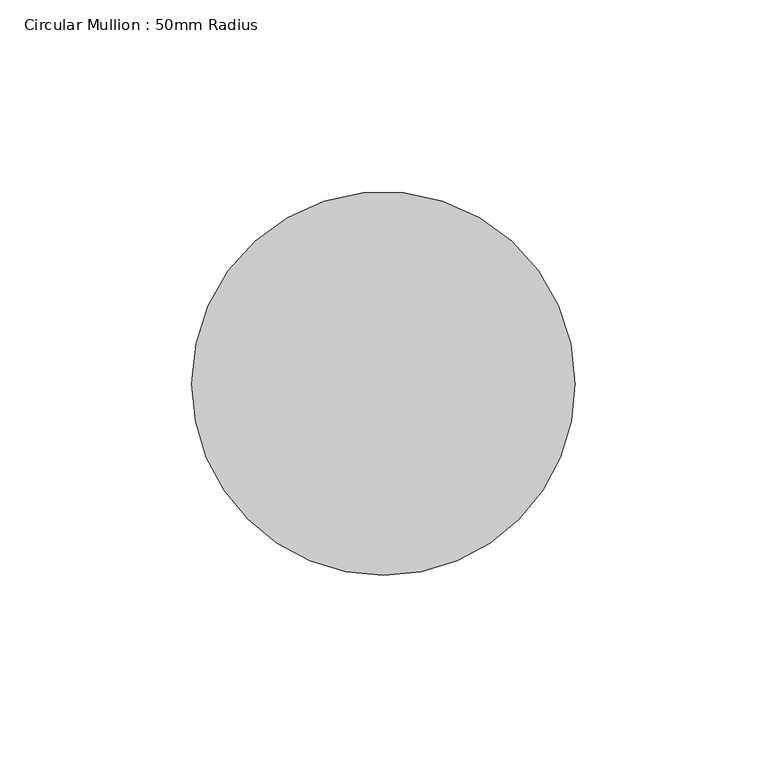
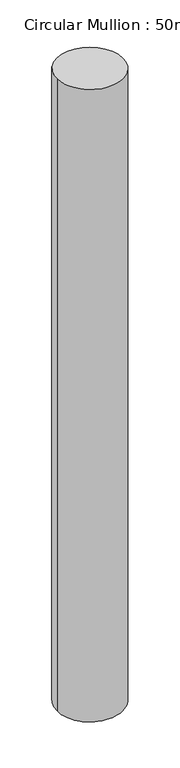
"""IFC4 building model written with IfcOpenShell, lengths in millimetres: member geometry, Circular Mullion : 50mm Radius."""

from ifc_helpers import new_model, si_unit, frame, origin, place, context, project, spatial, ellipse_curve, source, transform, mapped, element, save
from ifc_brep_helpers import plane_surface, cylinder_surface, advanced_brep


def circular_mullion_50mm_radius_8a95fe05(model_context):
    return source(origin(), model_context, "Body", "AdvancedBrep", [
        advanced_brep(
        [(-100.0, 0.0, 1.6217171), (0.0, 0.0, 0.0), (0.0, 0.0, -1012.0497266), (-100.0, 0.0, -1013.6442396)],
        [
            (0, 1, ellipse_curve(frame((-50.0, 0.0, 0.8108586), z_axis=(-0.01621331859733197, -0.014566336703536234, -0.9997624468518012), x_axis=(-0.7437023213754502, -0.6681555262929935, 0.021795638666932717)), 50.0118805, 50.0)),
            (1, 2),
            (2, 3, ellipse_curve(frame((-50.0, 0.0, -1012.8469831), z_axis=(-0.01594146823200777, -0.01432210145147921, 0.9997703471300905), x_axis=(0.7437081982268304, 0.6681608061618276, 0.021430188972056945)), 50.0114853, 50.0)),
            (3, 0),
            (1, 0, ellipse_curve(frame((-50.0, 0.0, 0.8108586), z_axis=(-0.01621331859733197, -0.014566336703536234, -0.9997624468518012), x_axis=(-0.7437023213754502, -0.6681555262929935, 0.021795638666932717)), 50.0118805, 50.0)),
            (3, 2, ellipse_curve(frame((-50.0, 0.0, -1012.8469831), z_axis=(-0.01594146823200777, -0.01432210145147921, 0.9997703471300905), x_axis=(0.7437081982268304, 0.6681608061618276, 0.021430188972056945)), 50.0114853, 50.0)),
        ],
        [
            cylinder_surface(frame((-50.0, 0.0, 0.0), z_axis=(0.0, 0.0, 1.0), x_axis=(1.0, 0.0, 0.0)), 50.0),
            plane_surface(frame((-203.7021945, 226.734329, 0.0), z_axis=(0.016213318597331973, 0.014566336703536237, 0.9997624468518014), x_axis=(0.7437023213754501, 0.6681555262929938, -0.02179563866693008))),
            plane_surface(frame((-203.7021945, 226.734329, -1012.0497266), z_axis=(0.01594146823200777, 0.01432210145147921, -0.9997703471300905), x_axis=(0.7437081982268302, 0.6681608061618275, 0.02143018897206872))),
        ],
        [
            (0, [[1, 2, 3, 4]]),
            (0, [[5, -4, 6, -2]]),
            (1, [[-1, -5]]),
            (2, [[-6, -3]]),
        ],
    ),
    ])


if __name__ == "__main__":
    model = new_model("IFC4")
    model_context = context("Model", 3, world=origin())
    ifc_project = project(units=[si_unit("LENGTHUNIT", "METRE", prefix="MILLI")], contexts=[model_context])
    site = spatial("IfcSite", under=ifc_project)
    building = spatial("IfcBuilding", under=site)
    placement = place(None, origin())
    circular_mullion_50mm_radius_shape = circular_mullion_50mm_radius_8a95fe05(model_context)
    element("IfcMember", 1, ObjectType="Circular Mullion : 50mm Radius", at=placement, inside=building, context=model_context, shape_type="MappedRepresentation", body=[
        mapped(circular_mullion_50mm_radius_shape, transform((0.0, 0.0, 0.0), x_axis=(1.0, 0.0, 0.0), y_axis=(0.0, 1.0, 0.0), z_axis=(0.0, 0.0, 1.0))),
    ])
    save(model, "model.ifc")

# Revit data of these elements
# Type "Circular Mullion : 50mm Radius"
#   built-in parameter 1007350 = 0.164042 (stored number, unit not read)
# Element 1 (IfcMember, "Circular Mullion : 50mm Radius")
#   Materials on its faces: "Aluminium"
# Materials
#   "Aluminium": class "Metal", colour RGB 247 247 247, transparency 0, Description = "Aluminium 6061", Cost = 0
